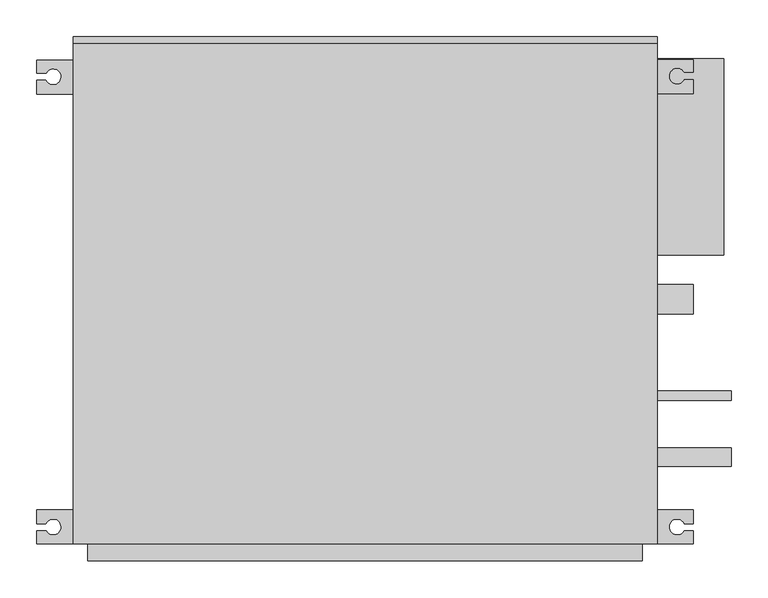
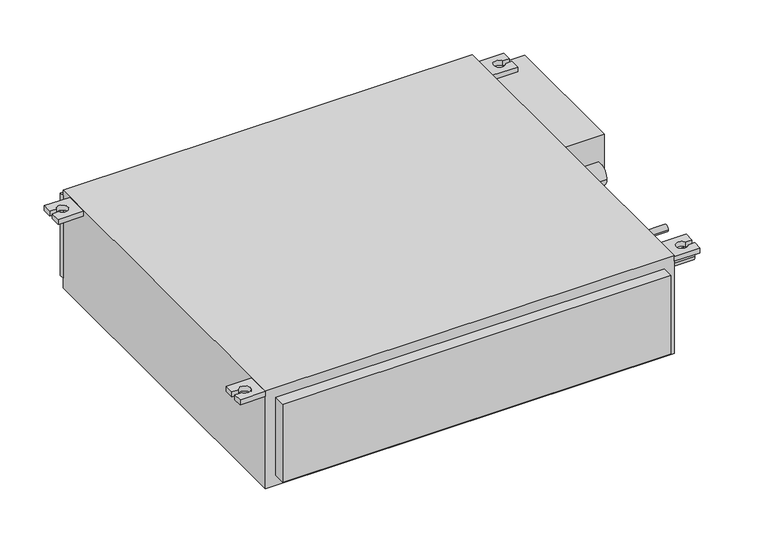
"""IFC4 building model written with IfcOpenShell, lengths in millimetres: proxy geometry, PEFY-P-NMSU-E_Low_Profile_Ducted : PEFY-P12NMSU-E."""

from ifc_helpers import new_model, si_unit, point, frame, frame_2d, origin, origin_with_axes, place, context, project, spatial, polyline, circle_curve, trimmed, segment, composite_curve, outline, extrude, source, transform, mapped, element, save


def mechanical_equipment_deea6110(model_context):
    return source(origin(), model_context, "Body", "SweptSolid", [
        extrude(outline(composite_curve([segment(polyline([(-444.2875, 282.0), (-444.2875, 300.9759165), (-432.1329311, 300.9759165)]), True, "CONTINUOUS"), segment(trimmed(circle_curve(frame_2d((-422.2738556, 305.4254582)), 10.8166442), [point((-432.1329311, 300.9759165))], [point((-431.8262803, 310.5))], True, "CARTESIAN"), True, "CONTINUOUS"), segment(polyline([(-431.8262803, 310.5), (-444.2875, 310.5), (-444.2875, 328.0), (-395.2875, 328.0), (-395.2875, 282.0), (-444.2875, 282.0)]), True, "CONTINUOUS")], self_intersect=False)), frame((0.0, 0.0, 188.55), z_axis=(0.0, 0.0, 1.0), x_axis=(1.0, 0.0, 0.0)), (0.0, 0.0, 1.0), 10.0),
        extrude(outline(composite_curve([segment(polyline([(-444.2875, -281.0), (-395.2875, -281.0), (-395.2875, -327.0), (-444.2875, -327.0), (-444.2875, -309.5), (-431.8262803, -309.5)]), True, "CONTINUOUS"), segment(trimmed(circle_curve(frame_2d((-422.2738556, -304.4254582)), 10.8166442), [point((-431.8262803, -309.5))], [point((-432.1329311, -299.9759165))], True, "CARTESIAN"), True, "CONTINUOUS"), segment(polyline([(-432.1329311, -299.9759165), (-444.2875, -299.9759165), (-444.2875, -281.0)]), True, "CONTINUOUS")], self_intersect=False)), frame((0.0, 0.0, 188.55), z_axis=(0.0, 0.0, 1.0), x_axis=(1.0, 0.0, 0.0)), (0.0, 0.0, 1.0), 10.0),
        extrude(outline(composite_curve([segment(polyline([(444.2875, 282.9429009), (395.2875, 282.9429009), (395.2875, 328.9429009), (444.2875, 328.9429009), (444.2875, 311.4429009), (431.8262803, 311.4429009)]), True, "CONTINUOUS"), segment(trimmed(circle_curve(frame_2d((422.2738556, 306.3683591)), 10.8166442), [point((431.8262803, 311.4429009))], [point((432.1329311, 301.9188174))], True, "CARTESIAN"), True, "CONTINUOUS"), segment(polyline([(432.1329311, 301.9188174), (444.2875, 301.9188174), (444.2875, 282.9429009)]), True, "CONTINUOUS")], self_intersect=False)), frame((0.0, 0.0, 188.55), z_axis=(0.0, 0.0, 1.0), x_axis=(1.0, 0.0, 0.0)), (0.0, 0.0, 1.0), 10.0),
        extrude(outline(composite_curve([segment(polyline([(444.2875, -281.0), (444.2875, -299.9759165), (432.1329311, -299.9759165)]), True, "CONTINUOUS"), segment(trimmed(circle_curve(frame_2d((422.2738556, -304.4254582)), 10.8166442), [point((432.1329311, -299.9759165))], [point((431.8262803, -309.5))], True, "CARTESIAN"), True, "CONTINUOUS"), segment(polyline([(431.8262803, -309.5), (444.2875, -309.5), (444.2875, -327.0), (395.2875, -327.0), (395.2875, -281.0), (444.2875, -281.0)]), True, "CONTINUOUS")], self_intersect=False)), frame((0.0, 0.0, 188.55), z_axis=(0.0, 0.0, 1.0), x_axis=(1.0, 0.0, 0.0)), (0.0, 0.0, 1.0), 10.0),
        extrude(outline(polyline([(395.2875, 350.04375), (-395.2875, 350.04375), (-395.2875, 359.5477547), (395.2875, 359.5477547), (395.2875, 350.04375)])), frame((0.0, 0.0, 20.0), z_axis=(0.0, 0.0, 1.0), x_axis=(1.0, 0.0, 0.0)), (0.0, 0.0, 1.0), 168.55),
        extrude(outline(composite_curve([segment(trimmed(circle_curve(frame_2d((4.0570991, 59.8)), 20.0421875), [point((-15.9850884, 59.8))], [point((24.0992866, 59.8))], False, "CARTESIAN"), True, "CONTINUOUS"), segment(trimmed(circle_curve(frame_2d((4.0570991, 59.8)), 20.0421875), [point((24.0992866, 59.8))], [point((-15.9850884, 59.8))], False, "CARTESIAN"), True, "CONTINUOUS")], self_intersect=False)), frame((395.2875, 0.0, 0.0), z_axis=(1.0, 0.0, 0.0), x_axis=(0.0, 1.0, 0.0)), (0.0, 0.0, 1.0), 26.9863556),
        extrude(outline(composite_curve([segment(trimmed(circle_curve(frame_2d((4.0570991, 149.6)), 20.0421875), [point((-15.9850884, 149.6))], [point((24.0992866, 149.6))], False, "CARTESIAN"), True, "CONTINUOUS"), segment(trimmed(circle_curve(frame_2d((4.0570991, 149.6)), 20.0421875), [point((24.0992866, 149.6))], [point((-15.9850884, 149.6))], False, "CARTESIAN"), True, "CONTINUOUS")], self_intersect=False)), frame((395.2875, 0.0, 0.0), z_axis=(1.0, 0.0, 0.0), x_axis=(0.0, 1.0, 0.0)), (0.0, 0.0, 1.0), 49.0),
        extrude(outline(composite_curve([segment(trimmed(circle_curve(frame_2d((-126.5596979, 100.0)), 6.4492188), [point((-133.0089166, 100.0))], [point((-120.1104791, 100.0))], False, "CARTESIAN"), True, "CONTINUOUS"), segment(trimmed(circle_curve(frame_2d((-126.5596979, 100.0)), 6.4492188), [point((-120.1104791, 100.0))], [point((-133.0089166, 100.0))], False, "CARTESIAN"), True, "CONTINUOUS")], self_intersect=False)), frame((395.2875, 0.0, 0.0), z_axis=(1.0, 0.0, 0.0), x_axis=(0.0, 1.0, 0.0)), (0.0, 0.0, 1.0), 100.0),
        extrude(outline(composite_curve([segment(trimmed(circle_curve(frame_2d((-209.7540575, 100.0)), 12.7), [point((-222.4540575, 100.0))], [point((-197.0540575, 100.0))], False, "CARTESIAN"), True, "CONTINUOUS"), segment(trimmed(circle_curve(frame_2d((-209.7540575, 100.0)), 12.7), [point((-197.0540575, 100.0))], [point((-222.4540575, 100.0))], False, "CARTESIAN"), True, "CONTINUOUS")], self_intersect=False)), frame((395.2875, 0.0, 0.0), z_axis=(1.0, 0.0, 0.0), x_axis=(0.0, 1.0, 0.0)), (0.0, 0.0, 1.0), 100.0),
        extrude(outline(polyline([(485.2875, 330.0), (485.2875, 64.0570991), (395.2875, 64.0570991), (395.2875, 330.0), (485.2875, 330.0)])), frame((0.0, 0.0, 20.0), z_axis=(0.0, 0.0, 1.0), x_axis=(1.0, 0.0, 0.0)), (0.0, 0.0, 1.0), 159.8),
        extrude(outline(polyline([(375.2875, -350.04375), (-375.2875, -350.04375), (-375.2875, -327.0), (375.2875, -327.0), (375.2875, -350.04375)])), frame((0.0, 0.0, 19.9585938), z_axis=(0.0, 0.0, 1.0), x_axis=(1.0, 0.0, 0.0)), (0.0, 0.0, 1.0), 159.8414063),
        extrude(outline(polyline([(-395.2875, -327.0), (-395.2875, 350.04375), (395.2875, 350.04375), (395.2875, -327.0), (-395.2875, -327.0)])), origin_with_axes(), (0.0, 0.0, 1.0), 200.0),
    ])


if __name__ == "__main__":
    model = new_model("IFC4")
    model_context = context("Model", 3, world=origin())
    ifc_project = project(units=[si_unit("LENGTHUNIT", "METRE", prefix="MILLI")], contexts=[model_context])
    site = spatial("IfcSite", under=ifc_project)
    building = spatial("IfcBuilding", under=site)
    placement = place(None, origin())
    mechanical_equipment_shape = mechanical_equipment_deea6110(model_context)
    element("IfcBuildingElementProxy", 1, Name="PEFY-P-NMSU-E_Low_Profile_Ducted : PEFY-P12NMSU-E", ObjectType="PEFY-P-NMSU-E_Low_Profile_Ducted : PEFY-P12NMSU-E", at=placement, inside=building, context=model_context, shape_type="MappedRepresentation", body=[
        mapped(mechanical_equipment_shape, transform((0.0, 0.0, 0.0), x_axis=(1.0, 0.0, 0.0), y_axis=(0.0, 1.0, 0.0), z_axis=(0.0, 0.0, 1.0))),
    ])
    save(model, "model.ifc")

# Revit data of these elements
# Type "PEFY-P-NMSU-E_Low_Profile_Ducted : PEFY-P12NMSU-E"
#   Subcategory = "HVAC"
#   Standard Air Filter = "Polypropylene Honeycomb"
#   Specification URL = "http://www.mrslim.com/customerCare/resources.asp"
#   Sound Pressure Levels (dB(A)) = "23-28-35"
#   SmartBIM Object Created By = "Reed Construction Data"
#   Refirigerant Pipe diameter (Liquid) = "1/4\""
#   Refirigerant Pipe diameter (Gas) = "1/2\""
#   Power Source = "208/230, 1, 60"
#   Power Consumption Heating = "0.05 kW"
#   Power Consumption Cooling = "0.07 kW"
#   Unit Weight (LBS) = "46"
#   Model = "PEFY-P12NMSU-E"
#   Manufacturer URL = "http://www.mrslim.com/customerCare/resources.asp"
#   Manufacturer = "Mitsubishi Electric"
#   Installation URL = "http://www.mrslim.com/customerCare/resources.asp"
#   Fan Motor Type = "DC Motor"
#   Fan Motor Output = "0.096 kW"
#   MCA = "0.68/0.74"
#   MOCP = "15 A"
#   E.S.P (In. W.G.) = ".02-.20"
#   Drainpipe Dimension = "1-1/4"
#   Description = "Ceiling Concealed Ducted Low Profile"
#   Condensate Lift Mechanism = "21-11/16\" "
#   Coil Type = "Cross Fin"
#   Heating Capacity (BTU) = "13500"
#   Fan Type x Quantity = "Sirocco Fan x 2"
#   Current Heating = "0.43 A"
#   Current Cooling = "0.53 A"
#   Cooling Capacity (BTU) = "12000"
#   Fan capacity (CFM) = "211-282-370 "
#   Assembly Code = "D3050200"
#   95 CSI = "15760"
#   04 CSI = "23 82 19 "
#   Width = 790.575 mm
#   Voltage = 0 V
#   Unit Supply Airflow [instance default] = 0 CFM
#   Unit Return Airflow [instance default] = 0 CFM
#   SmartBIM Object Version = 3
#   Height = 200 mm
#   Drain Pipe Radius = 20.042 mm
#   Depth = 700.088 mm
#   Default Elevation = 1219.2 mm
#   C = 888.575 mm
#   Brazing Connection Radius (Liquid) = 6.449 mm
#   Brazing Connection Radius (Gas) = 12.7 mm
#   Suspension Bolt Pitch = 842.575 mm
#   Apparent Load = 0 VA
#   Air Outlet Width = 750.575 mm
#   Air Inlet Width = 790.575 mm
#   Air Outlet Height = 159.841 mm
#   Air Inlet Height = 169 mm
#   Number of Poles = 1
#   Load Classification = Other
#   External Finish = Galvanized Steel Sheet
#   Air Outlet Unit Material = Metal Grill
#   Air Inlet Unit Material = Grill
#   URL = ""
# Element 1 (IfcBuildingElementProxy, "PEFY-P-NMSU-E_Low_Profile_Ducted : PEFY-P12NMSU-E")
#   Unit Supply Airflow = 460 CFM
#   Unit Return Airflow = 460 CFM
#   Materials on its faces: "Galvanized Steel Sheet", "Grill", "Metal Grill"
# Materials
#   "Galvanized Steel Sheet": class "Metal", colour RGB 189 187 185, transparency 0
#   "Metal Grill": class "Metal", colour RGB 10 10 10, transparency 0
#   "Grill": class "Plastic", colour RGB 5 5 5, transparency 0
